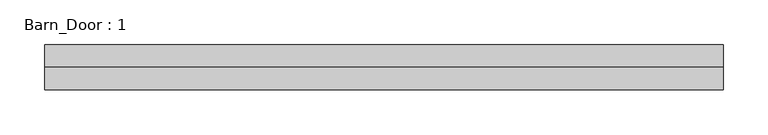
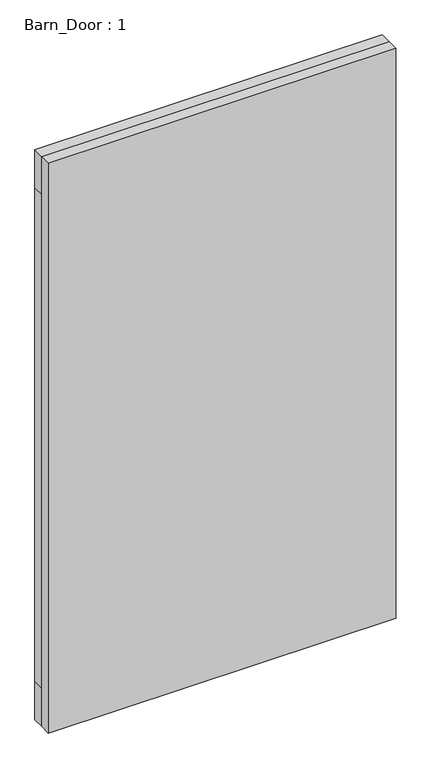
"""IFC4 building model written with IfcOpenShell, lengths in millimetres: proxy geometry, Barn_Door : 1."""

from ifc_helpers import new_model, si_unit, frame, origin, origin_with_axes, place, context, project, spatial, polyline, outline, extrude, source, transform, mapped, element, save


def barn_door_1_f580dd66(model_context):
    return source(origin(), model_context, "Body", "SweptSolid", [
        extrude(outline(polyline([(0.0, 134.9375), (-762.0, 134.9375), (-762.0, 160.3375), (0.0, 160.3375), (0.0, 134.9375)])), origin_with_axes(), (0.0, 0.0, 1.0), 1320.8),
        extrude(outline(polyline([(1134.231532, -88.9), (1231.9, -88.9), (1231.9, -138.8194392), (758.068468, -381.0), (1231.9, -623.1805608), (1231.9, -673.1), (1134.231532, -673.1), (660.4, -430.9194392), (186.568468, -673.1), (88.9, -673.1), (88.9, -623.1805608), (562.731532, -381.0), (88.9, -138.8194392), (88.9, -88.9), (186.568468, -88.9), (660.4, -331.0805608), (1134.231532, -88.9)])), frame((0.0, 160.3375, 0.0), z_axis=(0.0, 1.0, 0.0), x_axis=(0.0, 0.0, 1.0)), (0.0, 0.0, 1.0), 25.4),
        extrude(outline(polyline([(-673.1, 160.3375), (-762.0, 160.3375), (-762.0, 185.7375), (-673.1, 185.7375), (-673.1, 160.3375)])), frame((0.0, 0.0, 88.9), z_axis=(0.0, 0.0, 1.0), x_axis=(1.0, 0.0, 0.0)), (0.0, 0.0, 1.0), 1143.0),
        extrude(outline(polyline([(0.0, 160.3375), (-88.9, 160.3375), (-88.9, 185.7375), (0.0, 185.7375), (0.0, 160.3375)])), frame((0.0, 0.0, 88.9), z_axis=(0.0, 0.0, 1.0), x_axis=(1.0, 0.0, 0.0)), (0.0, 0.0, 1.0), 1143.0),
        extrude(outline(polyline([(0.0, 160.3375), (-762.0, 160.3375), (-762.0, 185.7375), (0.0, 185.7375), (0.0, 160.3375)])), frame((0.0, 0.0, 1231.9), z_axis=(0.0, 0.0, 1.0), x_axis=(1.0, 0.0, 0.0)), (0.0, 0.0, 1.0), 88.9),
        extrude(outline(polyline([(0.0, 160.3375), (-762.0, 160.3375), (-762.0, 185.7375), (0.0, 185.7375), (0.0, 160.3375)])), origin_with_axes(), (0.0, 0.0, 1.0), 88.9),
    ])


if __name__ == "__main__":
    model = new_model("IFC4")
    model_context = context("Model", 3, world=origin())
    ifc_project = project(units=[si_unit("LENGTHUNIT", "METRE", prefix="MILLI")], contexts=[model_context])
    site = spatial("IfcSite", under=ifc_project)
    building = spatial("IfcBuilding", under=site)
    placement = place(None, origin())
    barn_door_1_shape = barn_door_1_f580dd66(model_context)
    element("IfcBuildingElementProxy", 1, Name="Barn_Door : 1", ObjectType="Barn_Door : 1", at=placement, inside=building, context=model_context, shape_type="MappedRepresentation", body=[
        mapped(barn_door_1_shape, transform((0.0, 0.0, 0.0), x_axis=(1.0, 0.0, 0.0), y_axis=(0.0, 1.0, 0.0), z_axis=(0.0, 0.0, 1.0))),
    ])
    save(model, "model.ifc")

# Revit data of these elements
# Type "Barn_Door : 1"
#   Type Mark = "32"
#   Width = 2' - 6"
#   Rough Width = 0' - 0"
#   Height = 4' - 4"
#   Rail [instance default] = 5' - 0"
#   Frame Projection Ext. = 0' - 1"
#   Frame Width = 0' - 3 1/2"
#   Top Rail = DECORATIVE BARN DOOR
#   Door Framing = DECORATIVE BARN DOOR
#   Door = DECORATIVE BARN DOOR
#   Wall Closure = (empty or 0)
# Element 1 (IfcBuildingElementProxy, "Barn_Door : 1")
#   Materials on its faces: "DECORATIVE BARN DOOR"
# Materials
#   "DECORATIVE BARN DOOR": class "Generic", colour RGB 92 104 51, transparency 0, Cost = 0
